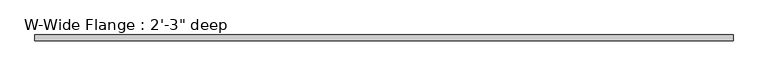
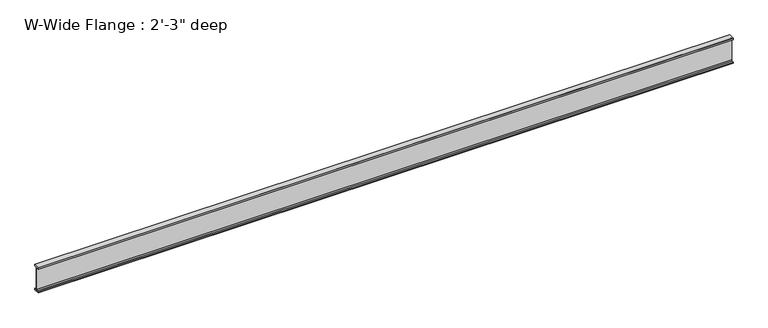
"""IFC4 building model written with IfcOpenShell, lengths in millimetres: beam geometry."""

import ifcopenshell
import ifcopenshell.guid

model = None  # the IFC model being written
_history = None  # IfcOwnerHistory: only IFC2X3 demands one
_inside = {}  # id of a spatial element -> (the spatial element, [elements in it])
_under = {}  # id of a project, library or spatial element -> (it, [spatial elements below it])
_declared = {}  # id of a project -> (the project, [libraries it declares])
_typed = {}  # id of a type object -> (the type object, [elements of that type])
_made_of = {}  # id of a material, layer set ... -> (it, [elements and type objects made of it])


def new_model(schema):
    """Start an empty IFC model of exactly this schema.

    Asked for "IFC4X3", IfcOpenShell would pick the latest addendum, in which some entities
    have other attributes; the version numbers below select the first issue.
    IFC2X3 requires an IfcOwnerHistory on every rooted entity: one is made here for all.
    """
    global model, _history
    if schema == "IFC4X3":
        model = ifcopenshell.file(schema_version=(4, 3, 0, 0))
    else:
        model = ifcopenshell.file(schema=schema)
    _inside.clear()
    _under.clear()
    _declared.clear()
    _typed.clear()
    _made_of.clear()
    _history = None
    if model.schema == "IFC2X3":
        org = make("IfcOrganization", Name="unknown")
        user = make(
            "IfcPersonAndOrganization",
            ThePerson=make("IfcPerson", FamilyName="unknown"),
            TheOrganization=org,
        )
        app = make(
            "IfcApplication",
            ApplicationDeveloper=org,
            Version="unknown",
            ApplicationFullName="unknown",
            ApplicationIdentifier="unknown",
        )
        _history = make(
            "IfcOwnerHistory",
            OwningUser=user,
            OwningApplication=app,
            ChangeAction="ADDED",
            CreationDate=0,
        )
    return model


def make(cls, **values):
    """One entity of the class cls with the attributes given. An attribute that is None is left unset."""
    return model.create_entity(
        cls, **{name: value for name, value in values.items() if value is not None}
    )


def rooted(cls, **values):
    """An entity with a GlobalId (a new one), such as an element, a storey or a relation."""
    return make(cls, GlobalId=ifcopenshell.guid.new(), OwnerHistory=_history, **values)


def si_unit(unit_type, name, prefix=None):
    """IfcSIUnit, for example si_unit("LENGTHUNIT", "METRE", prefix="MILLI")."""
    return make("IfcSIUnit", UnitType=unit_type, Prefix=prefix, Name=name)


def assignment(units):
    """IfcUnitAssignment: the units of a project."""
    return None if units is None else make("IfcUnitAssignment", Units=units)


def point(xyz):
    """IfcCartesianPoint."""
    return None if xyz is None else make("IfcCartesianPoint", Coordinates=xyz)


def direction(xyz):
    """IfcDirection."""
    return None if xyz is None else make("IfcDirection", DirectionRatios=xyz)


def frame(location, z_axis=None, x_axis=None):
    """IfcAxis2Placement3D, a coordinate frame: its origin and axes. An axis left out is left unset."""
    return make(
        "IfcAxis2Placement3D",
        Location=point(location),
        Axis=direction(z_axis),
        RefDirection=direction(x_axis),
    )


def frame_2d(location, x_axis=None):
    """IfcAxis2Placement2D, a coordinate frame in the plane: its origin and x axis."""
    return make(
        "IfcAxis2Placement2D", Location=point(location), RefDirection=direction(x_axis)
    )


def origin():
    """The frame at (0, 0, 0) with its axes left unset."""
    return frame((0.0, 0.0, 0.0))


def place(relative_to, where):
    """IfcLocalPlacement: puts the frame where relative to a parent placement (None: the world)."""
    return make(
        "IfcLocalPlacement", PlacementRelTo=relative_to, RelativePlacement=where
    )


def context(
    kind, dimensions, precision=None, world=None, true_north=None, identifier=None
):
    """IfcGeometricRepresentationContext, for example the 3D "Model" context."""
    return make(
        "IfcGeometricRepresentationContext",
        ContextIdentifier=identifier,
        ContextType=kind,
        CoordinateSpaceDimension=dimensions,
        Precision=precision,
        WorldCoordinateSystem=world,
        TrueNorth=true_north,
    )


def project(units=None, contexts=None):
    """IfcProject with its units and contexts."""
    return rooted(
        "IfcProject",
        Name="project",
        RepresentationContexts=contexts,
        UnitsInContext=assignment(units),
    )


def spatial(cls, under=None, at=None, **own):
    """A site, building, storey or space (cls), placed at a placement, below another one or the project."""
    s = rooted(cls, ObjectPlacement=at, **own)
    if under is not None:
        _under.setdefault(under.id(), (under, []))[1].append(s)
    return s


def polyline(points):
    """IfcPolyline through the points."""
    return make("IfcPolyline", Points=[point(p) for p in points])


def circle_curve(where, radius):
    """IfcCircle in the frame where."""
    return make("IfcCircle", Position=where, Radius=radius)


def trimmed(basis, trim1, trim2, sense, master):
    """IfcTrimmedCurve: the piece of a basis curve between two trims."""
    return make(
        "IfcTrimmedCurve",
        BasisCurve=basis,
        Trim1=trim1,
        Trim2=trim2,
        SenseAgreement=sense,
        MasterRepresentation=master,
    )


def segment(curve, same_sense, transition):
    """IfcCompositeCurveSegment."""
    return make(
        "IfcCompositeCurveSegment",
        Transition=transition,
        SameSense=same_sense,
        ParentCurve=curve,
    )


def composite_curve(segments, self_intersect=None):
    """IfcCompositeCurve: segments joined end to end."""
    return make("IfcCompositeCurve", Segments=segments, SelfIntersect=self_intersect)


def outline(outer, holes=None, kind="AREA"):
    """IfcArbitraryClosedProfileDef: a profile drawn as a closed curve; with holes, ...WithVoids."""
    if holes is None:
        return make("IfcArbitraryClosedProfileDef", ProfileType=kind, OuterCurve=outer)
    return make(
        "IfcArbitraryProfileDefWithVoids",
        ProfileType=kind,
        OuterCurve=outer,
        InnerCurves=holes,
    )


def extrude(swept, where, along, depth):
    """IfcExtrudedAreaSolid: the profile swept, set in the frame where, extruded along a direction by depth."""
    return make(
        "IfcExtrudedAreaSolid",
        SweptArea=swept,
        Position=where,
        ExtrudedDirection=direction(along),
        Depth=depth,
    )


def shape(context_of_items, identifier, shape_type, items):
    """IfcShapeRepresentation: the items that make up one representation, for example the "Body"."""
    return make(
        "IfcShapeRepresentation",
        ContextOfItems=context_of_items,
        RepresentationIdentifier=identifier,
        RepresentationType=shape_type,
        Items=items,
    )


def source(mapping_origin, context_of_items, identifier, shape_type, items):
    """IfcRepresentationMap: a shape defined once, which mapped items show again and again."""
    return make(
        "IfcRepresentationMap",
        MappingOrigin=mapping_origin,
        MappedRepresentation=shape(context_of_items, identifier, shape_type, items),
    )


def transform(
    local_origin,
    x_axis=None,
    y_axis=None,
    z_axis=None,
    scale=None,
    scale2=None,
    scale3=None,
    uniform=True,
):
    """IfcCartesianTransformationOperator3D, or its non-uniform kind. x_axis, y_axis, z_axis: its Axis1, 2, 3."""
    if uniform:
        return make(
            "IfcCartesianTransformationOperator3D",
            Axis1=direction(x_axis),
            Axis2=direction(y_axis),
            LocalOrigin=point(local_origin),
            Scale=scale,
            Axis3=direction(z_axis),
        )
    return make(
        "IfcCartesianTransformationOperator3DnonUniform",
        Axis1=direction(x_axis),
        Axis2=direction(y_axis),
        LocalOrigin=point(local_origin),
        Scale=scale,
        Axis3=direction(z_axis),
        Scale2=scale2,
        Scale3=scale3,
    )


def mapped(mapping_source, mapping_target):
    """IfcMappedItem: shows the shape of a source again, moved by a transform."""
    return make(
        "IfcMappedItem", MappingSource=mapping_source, MappingTarget=mapping_target
    )


def made_of(thing, what):
    """Note that an element or type object is made of a material, layer set ...; save() writes the relation."""
    if what is not None:
        _made_of.setdefault(what.id(), (what, []))[1].append(thing)
    return thing


def element(
    cls,
    number,
    at=None,
    inside=None,
    cuts=None,
    type_object=None,
    material=None,
    context=None,
    identifier="Body",
    shape_type=None,
    held_by="IfcProductDefinitionShape",
    body=None,
    shapes=None,
    **own,
):
    """One element of the class cls, such as IfcWall. Its Tag is "e" and its number.

    at: its placement. inside: the storey or other place that contains it. cuts: it is an
    opening in that element (IfcRelVoidsElement). A single representation is given by context,
    identifier, shape_type and body (its items); several are given by shapes. held_by: the class
    of the entity that holds the representations. save() writes the other relations.
    """
    e = rooted(cls, Tag="e%d" % number, ObjectPlacement=at, **own)
    if body is not None:
        shapes = [shape(context, identifier, shape_type, body)]
    if shapes is not None:
        e.Representation = make(held_by, Representations=shapes)
    if inside is not None:
        _inside.setdefault(inside.id(), (inside, []))[1].append(e)
    if cuts is not None:
        rooted(
            "IfcRelVoidsElement", RelatingBuildingElement=cuts, RelatedOpeningElement=e
        )
    if type_object is not None:
        _typed.setdefault(type_object.id(), (type_object, []))[1].append(e)
    return made_of(e, material)


def aggregate(whole, parts):
    """IfcRelAggregates: a whole, such as a stair, and the parts it consists of."""
    return rooted("IfcRelAggregates", RelatingObject=whole, RelatedObjects=parts)


def save(model, path):
    """Write the relations noted so far, then the file.

    IfcRelAggregates (storeys below a building ...), IfcRelContainedInSpatialStructure (elements
    in a storey), IfcRelDefinesByType, IfcRelAssociatesMaterial and IfcRelDeclares: one each for
    every whole, place, type object, material and project.
    """
    for whole, parts in _under.values():
        aggregate(whole, parts)
    for where, things in _inside.values():
        rooted(
            "IfcRelContainedInSpatialStructure",
            RelatedElements=things,
            RelatingStructure=where,
        )
    for kind, things in _typed.values():
        rooted("IfcRelDefinesByType", RelatedObjects=things, RelatingType=kind)
    for what, things in _made_of.values():
        rooted("IfcRelAssociatesMaterial", RelatedObjects=things, RelatingMaterial=what)
    for by, libraries in _declared.values():
        rooted("IfcRelDeclares", RelatingContext=by, RelatedDefinitions=libraries)
    model.write(path)


def beam_630f32b8(model_context):
    return source(origin(), model_context, "Body", "SweptSolid", [
        extrude(outline(composite_curve([segment(polyline([(76.2, -308.356), (76.2, -342.9), (-76.2, -342.9), (-76.2, -308.356), (-32.131, -308.356)]), True, "CONTINUOUS"), segment(trimmed(circle_curve(frame_2d((-32.131, -285.75)), 22.606), [point((-32.131, -308.356))], [point((-9.525, -285.75))], True, "CARTESIAN"), True, "CONTINUOUS"), segment(polyline([(-9.525, -285.75), (-9.525, 285.75)]), True, "CONTINUOUS"), segment(trimmed(circle_curve(frame_2d((-32.131, 285.75)), 22.606), [point((-9.525, 285.75))], [point((-32.131, 308.356))], True, "CARTESIAN"), True, "CONTINUOUS"), segment(polyline([(-32.131, 308.356), (-76.2, 308.356), (-76.2, 342.9), (76.2, 342.9), (76.2, 308.356), (32.131, 308.356)]), True, "CONTINUOUS"), segment(trimmed(circle_curve(frame_2d((32.131, 285.75)), 22.606), [point((32.131, 308.356))], [point((9.525, 285.75))], True, "CARTESIAN"), True, "CONTINUOUS"), segment(polyline([(9.525, 285.75), (9.525, -285.75)]), True, "CONTINUOUS"), segment(trimmed(circle_curve(frame_2d((32.131, -285.75)), 22.606), [point((9.525, -285.75))], [point((32.131, -308.356))], True, "CARTESIAN"), True, "CONTINUOUS"), segment(polyline([(32.131, -308.356), (76.2, -308.356)]), True, "CONTINUOUS")], self_intersect=False)), frame((-8971.3142226, 0.0, 0.0), z_axis=(1.0, 0.0, 0.0), x_axis=(0.0, 1.0, 0.0)), (0.0, 0.0, 1.0), 17938.4731374),
    ])


if __name__ == "__main__":
    model = new_model("IFC4")
    model_context = context("Model", 3, world=origin())
    ifc_project = project(units=[si_unit("LENGTHUNIT", "METRE", prefix="MILLI")], contexts=[model_context])
    site = spatial("IfcSite", under=ifc_project)
    building = spatial("IfcBuilding", under=site)
    placement = place(None, origin())
    beam_shape = beam_630f32b8(model_context)
    element("IfcBeam", 1, ObjectType="W-Wide Flange : 2'-3\" deep", at=placement, inside=building, context=model_context, shape_type="MappedRepresentation", body=[
        mapped(beam_shape, transform((0.0, 0.0, 0.0), x_axis=(1.0, 0.0, 0.0), y_axis=(0.0, 1.0, 0.0), z_axis=(0.0, 0.0, 1.0))),
    ])
    save(model, "model.ifc")

# Revit data of these elements
# Type "W-Wide Flange : 2'-3\" deep"
#   Assembly Code = "B10"
#   W = 166
#   Length [instance default] = 5' - 0"
#   bf = 0' - 6"
#   d = 2' - 3"
#   k = 0' - 2 1/4"
#   k2 = 0' - 0.89"
#   tf = 0' - 1.36"
#   tw = 0' - 0 3/4"
#   A = 0.338889 SF
#   Structural Material [instance default] = Steel ASTM A992
# Element 1 (IfcBeam, "W-Wide Flange : 2'-3\" deep")
#   Structural Material = STRUCTURAL STEEL - SEE STRUCT. DWGS
#   Materials on its faces: "STRUCTURAL STEEL - SEE STRUCT. DWGS"
# Materials
#   "Steel ASTM A992": class "Metal", colour RGB 199 199 199, transparency 0, Description = "Structural steel 50ksi", Cost = 0
#   "STRUCTURAL STEEL - SEE STRUCT. DWGS": class "Metal", colour RGB 137 146 153, transparency 0, Description = "Steel, mill finish", Cost = 0
